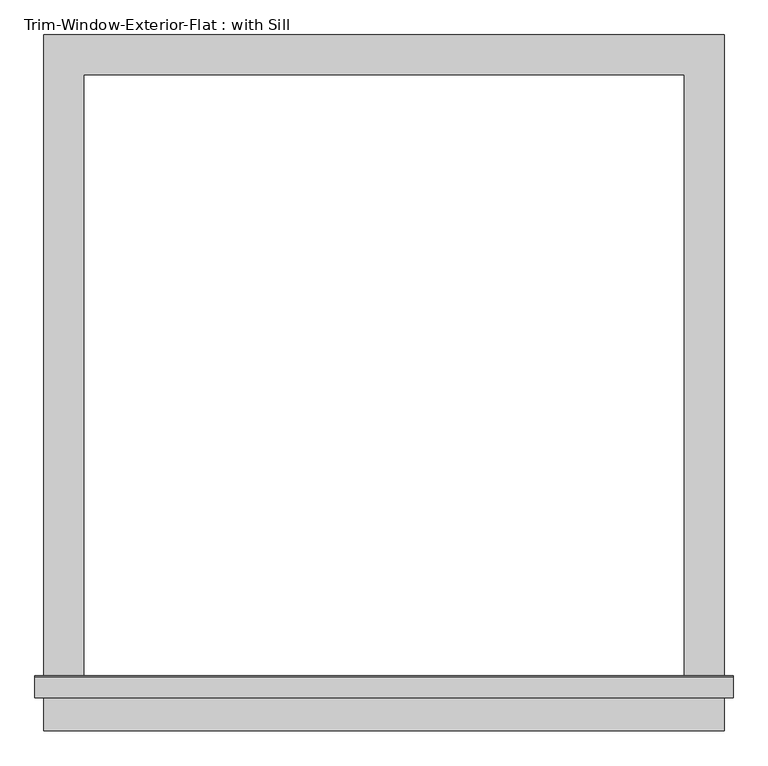
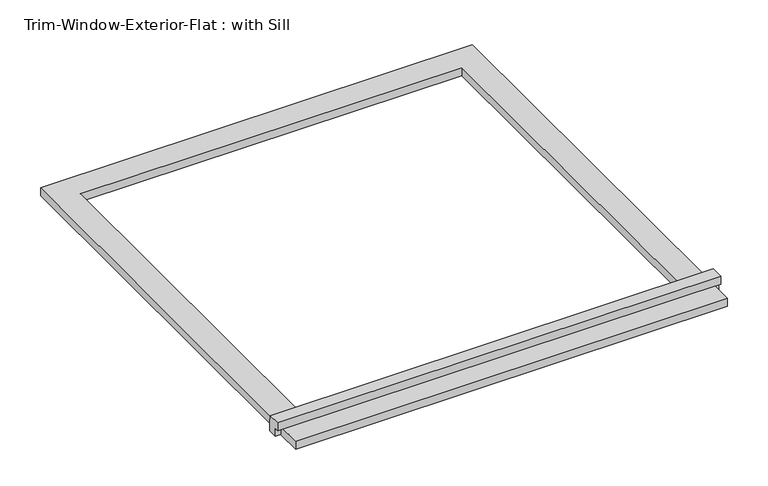
"""IFC4 building model written with IfcOpenShell, lengths in millimetres: proxy geometry, Trim-Window-Exterior-Flat : with Sill."""

from ifc_helpers import new_model, si_unit, frame, origin, origin_with_axes, place, context, project, spatial, polyline, outline, extrude, source, transform, mapped, element, save


def trim_window_exterior_flat_with_sill_a8480fd4(model_context):
    return source(origin(), model_context, "Body", "SweptSolid", [
        extrude(outline(polyline([(488.95, -885.7823709), (488.95, -942.9323709), (-488.95, -942.9323709), (-488.95, -885.7823709), (488.95, -885.7823709)])), origin_with_axes(), (0.0, 0.0, 1.0), 19.05),
        extrude(outline(polyline([(-895.35, 38.1), (-866.0580645, 38.1), (-863.6, 19.05), (-863.6, 0.0), (-885.7823709, 0.0), (-885.7823709, 19.05), (-895.35, 19.05), (-895.35, 38.1)])), frame((-501.65, 0.0, 0.0), z_axis=(1.0, 0.0, 0.0), x_axis=(0.0, 1.0, 0.0)), (0.0, 0.0, 1.0), 1003.3),
        extrude(outline(polyline([(-488.95, 57.15), (488.95, 57.15), (488.95, -863.6), (431.8, -863.6), (431.8, 0.0), (-431.8, 0.0), (-431.8, -863.6), (-488.95, -863.6), (-488.95, 57.15)])), origin_with_axes(), (0.0, 0.0, 1.0), 19.05),
    ])


if __name__ == "__main__":
    model = new_model("IFC4")
    model_context = context("Model", 3, world=origin())
    ifc_project = project(units=[si_unit("LENGTHUNIT", "METRE", prefix="MILLI")], contexts=[model_context])
    site = spatial("IfcSite", under=ifc_project)
    building = spatial("IfcBuilding", under=site)
    placement = place(None, origin())
    trim_window_exterior_flat_with_sill_shape = trim_window_exterior_flat_with_sill_a8480fd4(model_context)
    element("IfcBuildingElementProxy", 1, Name="Trim-Window-Exterior-Flat : with Sill", ObjectType="Trim-Window-Exterior-Flat : with Sill", at=placement, inside=building, context=model_context, shape_type="MappedRepresentation", body=[
        mapped(trim_window_exterior_flat_with_sill_shape, transform((0.0, 0.0, 0.0), x_axis=(1.0, 0.0, 0.0), y_axis=(0.0, 1.0, 0.0), z_axis=(0.0, 0.0, 1.0))),
    ])
    save(model, "model.ifc")

# Revit data of these elements
# Type "Trim-Window-Exterior-Flat : with Sill"
#   Trim Width = 0' - 2 1/4"
#   Trim Thickness_Picture Frame = 0' - 1 1/4"
#   Trim Thickness_with Sill = 0' - 0 3/4"
#   Sill Thickness = 0' - 1 1/4"
#   Opening Width [instance default] = 2' - 0"
#   Opening Height [instance default] = 3' - 0"
#   Default Elevation = 4' - 0"
#   Sill = yes
#   Picture Frame = no
#   Trim Material [instance default] = none
# Element 1 (IfcBuildingElementProxy, "Trim-Window-Exterior-Flat : with Sill")
#   Opening Width = 2' - 10"
#   Opening Height = 2' - 10"
#   Trim Material = 1X WOOD COMPOSITE TRIM
#   Materials on its faces: "1X WOOD COMPOSITE TRIM"
# Materials
#   "1X WOOD COMPOSITE TRIM": class "Generic", colour RGB 88 61 61, transparency 0, Cost = 0
